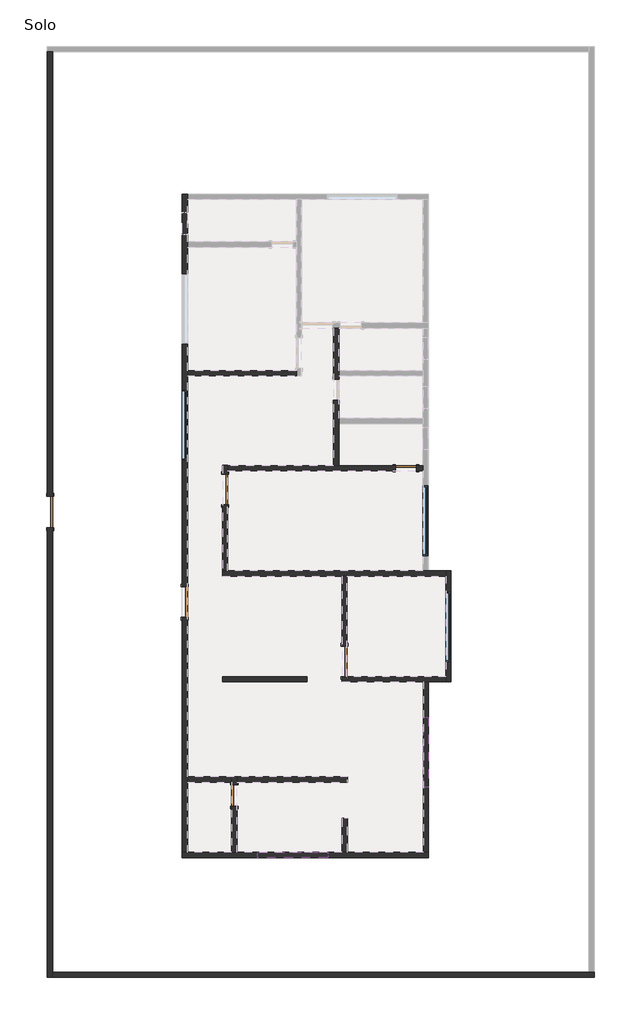
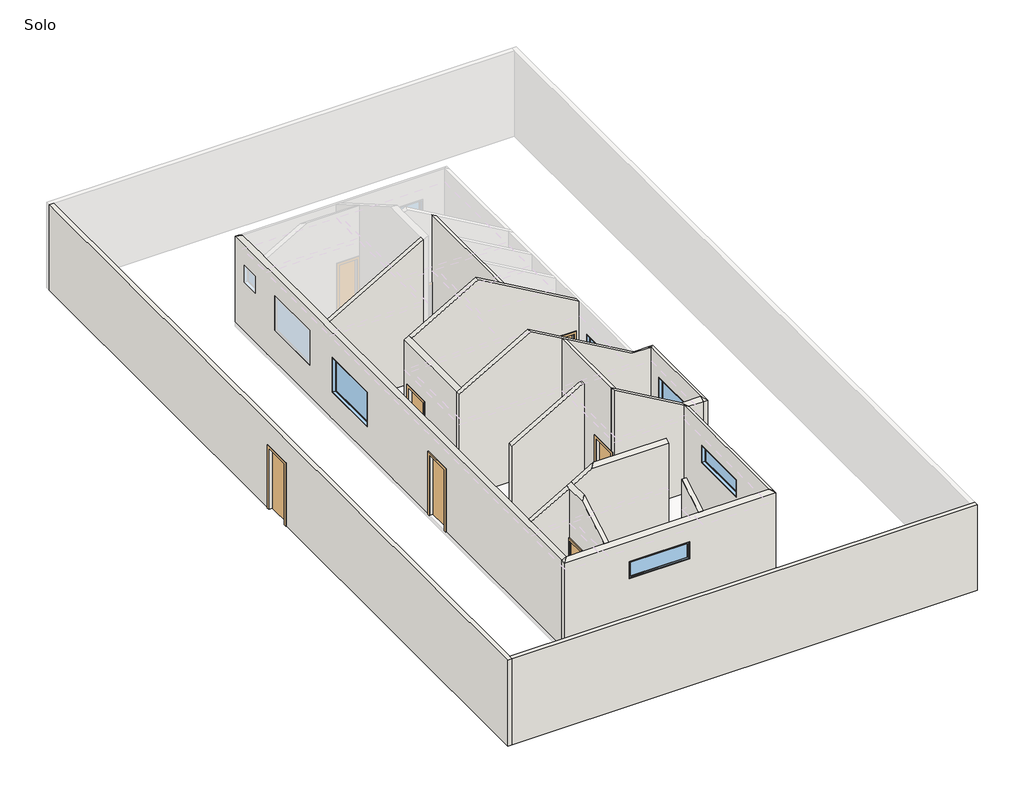
# One storey, part 1 of 2: 18 walls, 6 doors, 5 windows.
"""IFC4 building model written with IfcOpenShell, lengths in millimetres."""

import ifcopenshell
import ifcopenshell.guid

model = None  # the IFC model being written
_history = None  # IfcOwnerHistory: only IFC2X3 demands one
_inside = {}  # id of a spatial element -> (the spatial element, [elements in it])
_under = {}  # id of a project, library or spatial element -> (it, [spatial elements below it])
_declared = {}  # id of a project -> (the project, [libraries it declares])
_typed = {}  # id of a type object -> (the type object, [elements of that type])
_made_of = {}  # id of a material, layer set ... -> (it, [elements and type objects made of it])


def new_model(schema):
    """Start an empty IFC model of exactly this schema.

    Asked for "IFC4X3", IfcOpenShell would pick the latest addendum, in which some entities
    have other attributes; the version numbers below select the first issue.
    IFC2X3 requires an IfcOwnerHistory on every rooted entity: one is made here for all.
    """
    global model, _history
    if schema == "IFC4X3":
        model = ifcopenshell.file(schema_version=(4, 3, 0, 0))
    else:
        model = ifcopenshell.file(schema=schema)
    _inside.clear()
    _under.clear()
    _declared.clear()
    _typed.clear()
    _made_of.clear()
    _history = None
    if model.schema == "IFC2X3":
        org = make("IfcOrganization", Name="unknown")
        user = make(
            "IfcPersonAndOrganization",
            ThePerson=make("IfcPerson", FamilyName="unknown"),
            TheOrganization=org,
        )
        app = make(
            "IfcApplication",
            ApplicationDeveloper=org,
            Version="unknown",
            ApplicationFullName="unknown",
            ApplicationIdentifier="unknown",
        )
        _history = make(
            "IfcOwnerHistory",
            OwningUser=user,
            OwningApplication=app,
            ChangeAction="ADDED",
            CreationDate=0,
        )
    return model


def make(cls, **values):
    """One entity of the class cls with the attributes given. An attribute that is None is left unset."""
    return model.create_entity(
        cls, **{name: value for name, value in values.items() if value is not None}
    )


def rooted(cls, **values):
    """An entity with a GlobalId (a new one), such as an element, a storey or a relation."""
    return make(cls, GlobalId=ifcopenshell.guid.new(), OwnerHistory=_history, **values)


def si_unit(unit_type, name, prefix=None):
    """IfcSIUnit, for example si_unit("LENGTHUNIT", "METRE", prefix="MILLI")."""
    return make("IfcSIUnit", UnitType=unit_type, Prefix=prefix, Name=name)


def assignment(units):
    """IfcUnitAssignment: the units of a project."""
    return None if units is None else make("IfcUnitAssignment", Units=units)


def point(xyz):
    """IfcCartesianPoint."""
    return None if xyz is None else make("IfcCartesianPoint", Coordinates=xyz)


def direction(xyz):
    """IfcDirection."""
    return None if xyz is None else make("IfcDirection", DirectionRatios=xyz)


def frame(location, z_axis=None, x_axis=None):
    """IfcAxis2Placement3D, a coordinate frame: its origin and axes. An axis left out is left unset."""
    return make(
        "IfcAxis2Placement3D",
        Location=point(location),
        Axis=direction(z_axis),
        RefDirection=direction(x_axis),
    )


def origin():
    """The frame at (0, 0, 0) with its axes left unset."""
    return frame((0.0, 0.0, 0.0))


def origin_with_axes():
    """The frame at (0, 0, 0) with the z axis (0, 0, 1) and the x axis (1, 0, 0) written out."""
    return frame((0.0, 0.0, 0.0), z_axis=(0.0, 0.0, 1.0), x_axis=(1.0, 0.0, 0.0))


def place(relative_to, where):
    """IfcLocalPlacement: puts the frame where relative to a parent placement (None: the world)."""
    return make(
        "IfcLocalPlacement", PlacementRelTo=relative_to, RelativePlacement=where
    )


def context(
    kind, dimensions, precision=None, world=None, true_north=None, identifier=None
):
    """IfcGeometricRepresentationContext, for example the 3D "Model" context."""
    return make(
        "IfcGeometricRepresentationContext",
        ContextIdentifier=identifier,
        ContextType=kind,
        CoordinateSpaceDimension=dimensions,
        Precision=precision,
        WorldCoordinateSystem=world,
        TrueNorth=true_north,
    )


def project(units=None, contexts=None):
    """IfcProject with its units and contexts."""
    return rooted(
        "IfcProject",
        Name="project",
        RepresentationContexts=contexts,
        UnitsInContext=assignment(units),
    )


def spatial(cls, under=None, at=None, **own):
    """A site, building, storey or space (cls), placed at a placement, below another one or the project."""
    s = rooted(cls, ObjectPlacement=at, **own)
    if under is not None:
        _under.setdefault(under.id(), (under, []))[1].append(s)
    return s


def polyline(points):
    """IfcPolyline through the points."""
    return make("IfcPolyline", Points=[point(p) for p in points])


def outline(outer, holes=None, kind="AREA"):
    """IfcArbitraryClosedProfileDef: a profile drawn as a closed curve; with holes, ...WithVoids."""
    if holes is None:
        return make("IfcArbitraryClosedProfileDef", ProfileType=kind, OuterCurve=outer)
    return make(
        "IfcArbitraryProfileDefWithVoids",
        ProfileType=kind,
        OuterCurve=outer,
        InnerCurves=holes,
    )


def extrude(swept, where, along, depth):
    """IfcExtrudedAreaSolid: the profile swept, set in the frame where, extruded along a direction by depth."""
    return make(
        "IfcExtrudedAreaSolid",
        SweptArea=swept,
        Position=where,
        ExtrudedDirection=direction(along),
        Depth=depth,
    )


def faces_of(points, faces, orient=None, outer=None):
    """IfcFace entities. A face is a list of loops; a loop is a list of indices into points, from 0.

    orient and outer hold one flag for each loop. By default every Orientation is true, the
    first loop of a face is its IfcFaceOuterBound and the others are IfcFaceBound.
    """
    made = []
    for i, loops in enumerate(faces):
        bounds = []
        for j, loop in enumerate(loops):
            is_outer = j == 0 if outer is None else outer[i][j]
            bounds.append(
                make(
                    "IfcFaceOuterBound" if is_outer else "IfcFaceBound",
                    Bound=make("IfcPolyLoop", Polygon=[points[k] for k in loop]),
                    Orientation=True if orient is None else orient[i][j],
                )
            )
        made.append(make("IfcFace", Bounds=bounds))
    return made


def faceted_brep(points, faces, orient=None, outer=None, voids=None):
    """IfcFacetedBrep: a solid bounded by flat faces; with voids (closed shells), ...WithVoids."""
    shared = [point(p) for p in points]
    hull = make("IfcClosedShell", CfsFaces=faces_of(shared, faces, orient, outer))
    if voids is None:
        return make("IfcFacetedBrep", Outer=hull)
    return make(
        "IfcFacetedBrepWithVoids",
        Outer=hull,
        Voids=[
            make(cls, CfsFaces=faces_of(shared, fs, o, b)) for cls, fs, o, b in voids
        ],
    )


def shape(context_of_items, identifier, shape_type, items):
    """IfcShapeRepresentation: the items that make up one representation, for example the "Body"."""
    return make(
        "IfcShapeRepresentation",
        ContextOfItems=context_of_items,
        RepresentationIdentifier=identifier,
        RepresentationType=shape_type,
        Items=items,
    )


def source(mapping_origin, context_of_items, identifier, shape_type, items):
    """IfcRepresentationMap: a shape defined once, which mapped items show again and again."""
    return make(
        "IfcRepresentationMap",
        MappingOrigin=mapping_origin,
        MappedRepresentation=shape(context_of_items, identifier, shape_type, items),
    )


def transform(
    local_origin,
    x_axis=None,
    y_axis=None,
    z_axis=None,
    scale=None,
    scale2=None,
    scale3=None,
    uniform=True,
):
    """IfcCartesianTransformationOperator3D, or its non-uniform kind. x_axis, y_axis, z_axis: its Axis1, 2, 3."""
    if uniform:
        return make(
            "IfcCartesianTransformationOperator3D",
            Axis1=direction(x_axis),
            Axis2=direction(y_axis),
            LocalOrigin=point(local_origin),
            Scale=scale,
            Axis3=direction(z_axis),
        )
    return make(
        "IfcCartesianTransformationOperator3DnonUniform",
        Axis1=direction(x_axis),
        Axis2=direction(y_axis),
        LocalOrigin=point(local_origin),
        Scale=scale,
        Axis3=direction(z_axis),
        Scale2=scale2,
        Scale3=scale3,
    )


def mapped(mapping_source, mapping_target):
    """IfcMappedItem: shows the shape of a source again, moved by a transform."""
    return make(
        "IfcMappedItem", MappingSource=mapping_source, MappingTarget=mapping_target
    )


def made_of(thing, what):
    """Note that an element or type object is made of a material, layer set ...; save() writes the relation."""
    if what is not None:
        _made_of.setdefault(what.id(), (what, []))[1].append(thing)
    return thing


def element(
    cls,
    number,
    at=None,
    inside=None,
    cuts=None,
    type_object=None,
    material=None,
    context=None,
    identifier="Body",
    shape_type=None,
    held_by="IfcProductDefinitionShape",
    body=None,
    shapes=None,
    **own,
):
    """One element of the class cls, such as IfcWall. Its Tag is "e" and its number.

    at: its placement. inside: the storey or other place that contains it. cuts: it is an
    opening in that element (IfcRelVoidsElement). A single representation is given by context,
    identifier, shape_type and body (its items); several are given by shapes. held_by: the class
    of the entity that holds the representations. save() writes the other relations.
    """
    e = rooted(cls, Tag="e%d" % number, ObjectPlacement=at, **own)
    if body is not None:
        shapes = [shape(context, identifier, shape_type, body)]
    if shapes is not None:
        e.Representation = make(held_by, Representations=shapes)
    if inside is not None:
        _inside.setdefault(inside.id(), (inside, []))[1].append(e)
    if cuts is not None:
        rooted(
            "IfcRelVoidsElement", RelatingBuildingElement=cuts, RelatedOpeningElement=e
        )
    if type_object is not None:
        _typed.setdefault(type_object.id(), (type_object, []))[1].append(e)
    return made_of(e, material)


def aggregate(whole, parts):
    """IfcRelAggregates: a whole, such as a stair, and the parts it consists of."""
    return rooted("IfcRelAggregates", RelatingObject=whole, RelatedObjects=parts)


def save(model, path):
    """Write the relations noted so far, then the file.

    IfcRelAggregates (storeys below a building ...), IfcRelContainedInSpatialStructure (elements
    in a storey), IfcRelDefinesByType, IfcRelAssociatesMaterial and IfcRelDeclares: one each for
    every whole, place, type object, material and project.
    """
    for whole, parts in _under.values():
        aggregate(whole, parts)
    for where, things in _inside.values():
        rooted(
            "IfcRelContainedInSpatialStructure",
            RelatedElements=things,
            RelatingStructure=where,
        )
    for kind, things in _typed.values():
        rooted("IfcRelDefinesByType", RelatedObjects=things, RelatingType=kind)
    for what, things in _made_of.values():
        rooted("IfcRelAssociatesMaterial", RelatedObjects=things, RelatingMaterial=what)
    for by, libraries in _declared.values():
        rooted("IfcRelDeclares", RelatingContext=by, RelatedDefinitions=libraries)
    model.write(path)


def door_0762_x_2032mm_f712f77f(model_context):
    return source(origin(), model_context, "Body", "SweptSolid", [
        extrude(outline(polyline([(2108.0, -376.0), (0.0, -376.0), (0.0, -300.0), (2032.0, -300.0), (2032.0, 300.0), (0.0, 300.0), (0.0, 376.0), (2108.0, 376.0), (2108.0, -376.0)])), frame((0.0, 75.0, 0.0), z_axis=(0.0, 1.0, 0.0), x_axis=(0.0, 0.0, 1.0)), (0.0, 0.0, 1.0), 25.0),
        extrude(outline(polyline([(2108.0, 376.0), (2108.0, -376.0), (0.0, -376.0), (0.0, -300.0), (2032.0, -300.0), (2032.0, 300.0), (0.0, 300.0), (0.0, 376.0), (2108.0, 376.0)])), frame((0.0, -100.0, 0.0), z_axis=(0.0, 1.0, 0.0), x_axis=(0.0, 0.0, 1.0)), (0.0, 0.0, 1.0), 25.0),
        extrude(outline(polyline([(300.0, 24.0), (-300.0, 24.0), (-300.0, 75.0), (300.0, 75.0), (300.0, 24.0)])), origin_with_axes(), (0.0, 0.0, 1.0), 2032.0),
    ])


def door_0864_x_2134mm_0748c0c9(model_context):
    return source(origin(), model_context, "Body", "SweptSolid", [
        extrude(outline(polyline([(2210.0, -508.0), (0.0, -508.0), (0.0, -432.0), (2134.0, -432.0), (2134.0, 432.0), (0.0, 432.0), (0.0, 508.0), (2210.0, 508.0), (2210.0, -508.0)])), frame((0.0, -100.0, 0.0), z_axis=(0.0, 1.0, 0.0), x_axis=(0.0, 0.0, 1.0)), (0.0, 0.0, 1.0), 25.0),
        extrude(outline(polyline([(2210.0, 508.0), (2210.0, -508.0), (0.0, -508.0), (0.0, -432.0), (2134.0, -432.0), (2134.0, 432.0), (0.0, 432.0), (0.0, 508.0), (2210.0, 508.0)])), frame((0.0, 75.0, 0.0), z_axis=(0.0, 1.0, 0.0), x_axis=(0.0, 0.0, 1.0)), (0.0, 0.0, 1.0), 25.0),
        extrude(outline(polyline([(432.0, -24.0), (432.0, -75.0), (-432.0, -75.0), (-432.0, -24.0), (432.0, -24.0)])), origin_with_axes(), (0.0, 0.0, 1.0), 2134.0),
    ])


def door_0864_x_2134mm_191ab4f9(model_context):
    return source(origin(), model_context, "Body", "SweptSolid", [
        extrude(outline(polyline([(2210.0, -508.0), (0.0, -508.0), (0.0, -432.0), (2134.0, -432.0), (2134.0, 432.0), (0.0, 432.0), (0.0, 508.0), (2210.0, 508.0), (2210.0, -508.0)])), frame((0.0, 75.0, 0.0), z_axis=(0.0, 1.0, 0.0), x_axis=(0.0, 0.0, 1.0)), (0.0, 0.0, 1.0), 25.0),
        extrude(outline(polyline([(2210.0, 508.0), (2210.0, -508.0), (0.0, -508.0), (0.0, -432.0), (2134.0, -432.0), (2134.0, 432.0), (0.0, 432.0), (0.0, 508.0), (2210.0, 508.0)])), frame((0.0, -100.0, 0.0), z_axis=(0.0, 1.0, 0.0), x_axis=(0.0, 0.0, 1.0)), (0.0, 0.0, 1.0), 25.0),
        extrude(outline(polyline([(432.0, 24.0), (-432.0, 24.0), (-432.0, 75.0), (432.0, 75.0), (432.0, 24.0)])), origin_with_axes(), (0.0, 0.0, 1.0), 2134.0),
    ])


def door_0915_x_2134mm_ecbf01f7(model_context):
    return source(origin(), model_context, "Body", "SweptSolid", [
        extrude(outline(polyline([(2210.0, -526.0), (0.0, -526.0), (0.0, -450.0), (2134.0, -450.0), (2134.0, 450.0), (0.0, 450.0), (0.0, 526.0), (2210.0, 526.0), (2210.0, -526.0)])), frame((0.0, 75.0, 0.0), z_axis=(0.0, 1.0, 0.0), x_axis=(0.0, 0.0, 1.0)), (0.0, 0.0, 1.0), 25.0),
        extrude(outline(polyline([(2210.0, 526.0), (2210.0, -526.0), (0.0, -526.0), (0.0, -450.0), (2134.0, -450.0), (2134.0, 450.0), (0.0, 450.0), (0.0, 526.0), (2210.0, 526.0)])), frame((0.0, -100.0, 0.0), z_axis=(0.0, 1.0, 0.0), x_axis=(0.0, 0.0, 1.0)), (0.0, 0.0, 1.0), 25.0),
        extrude(outline(polyline([(450.0, 24.0), (-450.0, 24.0), (-450.0, 75.0), (450.0, 75.0), (450.0, 24.0)])), origin_with_axes(), (0.0, 0.0, 1.0), 2134.0),
    ])


def m_fixo_0915_x_0610mm_568dc35f(model_context):
    return source(origin(), model_context, "Body", "SweptSolid", [
        extrude(outline(polyline([(-937.0, 53.0), (937.0, 53.0), (937.0, 41.0), (-937.0, 41.0), (-937.0, 53.0)])), frame((0.0, 0.0, 2063.0), z_axis=(0.0, 0.0, 1.0), x_axis=(1.0, 0.0, 0.0)), (0.0, 0.0, 1.0), 484.0),
        extrude(outline(polyline([(2591.0, -981.0), (2019.0, -981.0), (2019.0, 981.0), (2591.0, 981.0), (2591.0, -981.0)]), holes=[polyline([(2547.0, -937.0), (2547.0, 937.0), (2063.0, 937.0), (2063.0, -937.0), (2547.0, -937.0)])]), frame((0.0, 25.0, 0.0), z_axis=(0.0, 1.0, 0.0), x_axis=(0.0, 0.0, 1.0)), (0.0, 0.0, 1.0), 44.0),
        extrude(outline(polyline([(2610.0, -1000.0), (2000.0, -1000.0), (2000.0, 1000.0), (2610.0, 1000.0), (2610.0, -1000.0)]), holes=[polyline([(2591.0, -981.0), (2591.0, 981.0), (2019.0, 981.0), (2019.0, -981.0), (2591.0, -981.0)])]), frame((0.0, 25.0, 0.0), z_axis=(0.0, 1.0, 0.0), x_axis=(0.0, 0.0, 1.0)), (0.0, 0.0, 1.0), 63.0),
        extrude(outline(polyline([(2610.0, -1000.0), (2000.0, -1000.0), (2000.0, 1000.0), (2610.0, 1000.0), (2610.0, -1000.0)]), holes=[polyline([(2578.0, -968.0), (2578.0, 968.0), (2032.0, 968.0), (2032.0, -968.0), (2578.0, -968.0)])]), frame((0.0, -62.0, 0.0), z_axis=(0.0, 1.0, 0.0), x_axis=(0.0, 0.0, 1.0)), (0.0, 0.0, 1.0), 87.0),
    ])


def m_fixo_0915_x_1220mm_8e554ddc(model_context):
    return source(origin(), model_context, "Body", "SweptSolid", [
        extrude(outline(polyline([(-937.0, 53.0), (937.0, 53.0), (937.0, 41.0), (-937.0, 41.0), (-937.0, 53.0)])), frame((0.0, 0.0, 978.0), z_axis=(0.0, 0.0, 1.0), x_axis=(1.0, 0.0, 0.0)), (0.0, 0.0, 1.0), 1094.0),
        extrude(outline(polyline([(2116.0, -981.0), (934.0, -981.0), (934.0, 981.0), (2116.0, 981.0), (2116.0, -981.0)]), holes=[polyline([(2072.0, -937.0), (2072.0, 937.0), (978.0, 937.0), (978.0, -937.0), (2072.0, -937.0)])]), frame((0.0, 25.0, 0.0), z_axis=(0.0, 1.0, 0.0), x_axis=(0.0, 0.0, 1.0)), (0.0, 0.0, 1.0), 44.0),
        extrude(outline(polyline([(2135.0, -1000.0), (915.0, -1000.0), (915.0, 1000.0), (2135.0, 1000.0), (2135.0, -1000.0)]), holes=[polyline([(2116.0, -981.0), (2116.0, 981.0), (934.0, 981.0), (934.0, -981.0), (2116.0, -981.0)])]), frame((0.0, 25.0, 0.0), z_axis=(0.0, 1.0, 0.0), x_axis=(0.0, 0.0, 1.0)), (0.0, 0.0, 1.0), 63.0),
        extrude(outline(polyline([(2135.0, -1000.0), (915.0, -1000.0), (915.0, 1000.0), (2135.0, 1000.0), (2135.0, -1000.0)]), holes=[polyline([(2103.0, -968.0), (2103.0, 968.0), (947.0, 968.0), (947.0, -968.0), (2103.0, -968.0)])]), frame((0.0, -62.0, 0.0), z_axis=(0.0, 1.0, 0.0), x_axis=(0.0, 0.0, 1.0)), (0.0, 0.0, 1.0), 87.0),
    ])


model = new_model("IFC4")

# Units and contexts
model_context = context("Model", 3, world=origin())
ifc_project = project(units=[si_unit("LENGTHUNIT", "METRE", prefix="MILLI")], contexts=[model_context])

# Site, building, storey
site = spatial("IfcSite", under=ifc_project)
building = spatial("IfcBuilding", under=site)
storey = spatial("IfcBuildingStorey", under=building, Name="Solo", Elevation=0.0)

# Doors
placement = place(None, origin())
door_0762_x_2032mm_shape = door_0762_x_2032mm_f712f77f(model_context)
element("IfcDoor", 1, ObjectType="M_Folha única : 0762 x 2032mm", at=placement, inside=storey, context=model_context, shape_type="MappedRepresentation", body=[
    mapped(door_0762_x_2032mm_shape, transform((-4950.9149651, -8006.6262329, 0.0), x_axis=(0.0, 1.0, 0.0), y_axis=(-1.0, 0.0, 0.0), z_axis=(0.0, 0.0, 1.0))),
])
element("IfcDoor", 2, ObjectType="M_Folha única : 0762 x 2032mm", at=placement, inside=storey, context=model_context, shape_type="MappedRepresentation", body=[
    mapped(door_0762_x_2032mm_shape, transform((-70.8698769, 1295.0972582, 0.0), x_axis=(1.0, 0.0, 0.0), y_axis=(0.0, 1.0, 0.0), z_axis=(0.0, 0.0, 1.0))),
])
door_0864_x_2134mm_shape = door_0864_x_2134mm_0748c0c9(model_context)
element("IfcDoor", 3, ObjectType="M_Folha única : 0864 x 2134mm", at=placement, inside=storey, context=model_context, shape_type="MappedRepresentation", body=[
    mapped(door_0864_x_2134mm_shape, transform((-5214.335632, 688.0972582, 0.0), x_axis=(0.0, 1.0, 0.0), y_axis=(-1.0, 0.0, 0.0), z_axis=(0.0, 0.0, 1.0))),
])
element("IfcDoor", 4, ObjectType="M_Folha única : 0864 x 2134mm", at=placement, inside=storey, context=model_context, shape_type="MappedRepresentation", body=[
    mapped(door_0864_x_2134mm_shape, transform((-6360.8698767, -2511.9027414, 0.0), x_axis=(0.0, 1.0, 0.0), y_axis=(-1.0, 0.0, 0.0), z_axis=(0.0, 0.0, 1.0))),
])
door_0864_x_2134mm_2_shape = door_0864_x_2134mm_191ab4f9(model_context)
element("IfcDoor", 5, ObjectType="M_Folha única : 0864 x 2134mm", at=placement, inside=storey, context=model_context, shape_type="MappedRepresentation", body=[
    mapped(door_0864_x_2134mm_2_shape, transform((-1820.8247891, -4192.9027402, 0.0), x_axis=(0.0, -1.0, 0.0), y_axis=(1.0, 0.0, 0.0), z_axis=(0.0, 0.0, 1.0))),
])
door_0915_x_2134mm_shape = door_0915_x_2134mm_ecbf01f7(model_context)
element("IfcDoor", 6, ObjectType="M_Folha única : 0915 x 2134mm", at=placement, inside=storey, context=model_context, shape_type="MappedRepresentation", body=[
    mapped(door_0915_x_2134mm_shape, transform((-10190.8698769, 50.0972598, 0.0), x_axis=(0.0, -1.0, 0.0), y_axis=(1.0, 0.0, 0.0), z_axis=(0.0, 0.0, 1.0))),
])

# Walls
element("IfcWall", 7, ObjectType="Genérico - 140 mm Alvenaria", at=placement, inside=storey, context=model_context, shape_type="Brep", body=[
    faceted_brep([(574.1301232, -9623.7945276, 0.0), (424.1301232, -9623.7945276, 0.0), (-1735.8698771, -9623.7945276, 0.0), (-1885.8698771, -9623.7945276, 0.0), (-4875.9149651, -9623.7945276, 0.0), (-5025.9149651, -9623.7945276, 0.0), (-6285.8698767, -9623.7945276, 0.0), (-6435.8698767, -9623.7945276, 0.0), (-6435.8698767, -9623.7945276, 3000.0), (-6285.8698767, -9623.7945276, 3086.6025404), (-5025.9149651, -9623.7945276, 3086.6025404), (-4875.9149651, -9623.7945276, 3086.6025404), (-1885.8698771, -9623.7945276, 3086.6025404), (-1735.8698771, -9623.7945276, 3086.6025404), (424.1301232, -9623.7945276, 3086.6025404), (574.1301232, -9623.7945276, 3000.0), (-2285.8698771, -9623.7945276, 1690.0), (-2285.8698771, -9623.7945276, 2300.0), (-4285.8698771, -9623.7945276, 2300.0), (-4285.8698771, -9623.7945276, 1690.0), (574.1301232, -9773.7945276, 0.0), (574.1301232, -9773.7945276, 3000.0), (-6435.8698767, -9773.7945276, 3000.0), (-6435.8698767, -9773.7945276, 0.0), (-2285.8698771, -9773.7945276, 1690.0), (-4285.8698771, -9773.7945276, 1690.0), (-4285.8698771, -9773.7945276, 2300.0), (-2285.8698771, -9773.7945276, 2300.0)], [[[0, 1, 2, 3, 4, 5, 6, 7, 8, 9, 10, 11, 12, 13, 14, 15], [16, 17, 18, 19]], [[20, 21, 22, 23], [24, 25, 26, 27]], [[7, 6, 5, 4, 3, 2, 1, 0, 20, 23]], [[8, 7, 23, 22]], [[0, 15, 21, 20]], [[17, 16, 24, 27]], [[18, 17, 27, 26]], [[19, 18, 26, 25]], [[16, 19, 25, 24]], [[15, 14, 21]], [[14, 13, 12, 11, 10, 9, 22, 21]], [[9, 8, 22]]]),
])
element("IfcWall", 8, ObjectType="Genérico - 140 mm Alvenaria", at=placement, inside=storey, context=model_context, shape_type="Brep", body=[
    faceted_brep([(-5025.9149651, -7474.9027402, 0.0), (-5025.9149651, -7476.6262329, 0.0), (-5025.9149651, -7626.6262329, 0.0), (-5025.9149651, -7706.6262329, 0.0), (-5025.9149651, -7706.6262329, 2032.0), (-5025.9149651, -8306.6262329, 2032.0), (-5025.9149651, -8306.6262329, 0.0), (-5025.9149651, -9623.7945276, 0.0), (-5025.9149651, -9623.7945276, 3086.6025404), (-5025.9149651, -8363.839616, 3814.0378477), (-5025.9149651, -7626.6262329, 3814.0378477), (-5025.9149651, -7476.6262329, 3814.0378477), (-5025.9149651, -7474.9027402, 3814.0378477), (-4875.9149651, -7706.6262329, 2032.0), (-4875.9149651, -7706.6262329, 0.0), (-4875.9149651, -7626.6262329, 0.0), (-4875.9149651, -7476.6262329, 0.0), (-4875.9149651, -7474.9027402, 0.0), (-4875.9149651, -7474.9027402, 3900.6403881), (-4875.9149651, -7476.6262329, 3900.6403881), (-4875.9149651, -7626.6262329, 3900.6403881), (-4875.9149651, -8213.839616, 3900.6403881), (-4875.9149651, -9623.7945276, 3086.6025404), (-4875.9149651, -9623.7945276, 0.0), (-4875.9149651, -8306.6262329, 0.0), (-4875.9149651, -8306.6262329, 2032.0)], [[[0, 1, 2, 3, 4, 5, 6, 7, 8, 9, 10, 11, 12]], [[13, 14, 15, 16, 17, 18, 19, 20, 21, 22, 23, 24, 25]], [[24, 23, 7, 6]], [[17, 16, 15, 14, 3, 2, 1, 0]], [[0, 12, 18, 17]], [[8, 7, 23, 22]], [[4, 3, 14, 13]], [[5, 4, 13, 25]], [[6, 5, 25, 24]], [[12, 11, 10, 9, 21, 20, 19, 18]], [[9, 8, 22, 21]]]),
])
element("IfcWall", 9, ObjectType="Genérico - 140 mm Alvenaria", at=placement, inside=storey, context=model_context, shape_type="Brep", body=[
    faceted_brep([(-4875.9149651, -7626.6262329, 0.0), (-1735.8698771, -7626.6262329, 0.0), (-1735.8698771, -7626.6262329, 4239.6681929), (-4288.7015821, -7626.6262329, 4239.6681929), (-4875.9149651, -7626.6262329, 3900.6403881), (-4875.9149651, -7476.6262329, 0.0), (-4875.9149651, -7476.6262329, 3900.6403881), (-4138.7015821, -7476.6262329, 4326.2707333), (-1735.8698771, -7476.6262329, 4326.2707333), (-1735.8698771, -7476.6262329, 0.0)], [[[0, 1, 2, 3, 4]], [[5, 6, 7, 8, 9]], [[1, 0, 5, 9]], [[2, 1, 9, 8]], [[0, 4, 6, 5]], [[4, 3, 7, 6]], [[3, 2, 8, 7]]]),
])
element("IfcWall", 10, ObjectType="Genérico - 140 mm Alvenaria", at=placement, inside=storey, context=model_context, shape_type="SweptSolid", body=[
    extrude(outline(polyline([(-8644.9027402, 0.0), (-9623.7945276, 0.0), (-9623.7945276, 3086.6025404), (-8644.9027402, 3651.7659773), (-8644.9027402, 0.0)])), frame((-1885.8698771, 0.0, 0.0), z_axis=(1.0, 0.0, 0.0), x_axis=(0.0, 1.0, 0.0)), (0.0, 0.0, 1.0), 150.0),
])
element("IfcWall", 11, ObjectType="Genérico - 140 mm Alvenaria", at=placement, inside=storey, context=model_context, shape_type="SweptSolid", body=[
    extrude(outline(polyline([(0.0, -6285.8698767), (0.0, -5025.9149651), (3814.0378477, -5025.9149651), (3086.6025404, -6285.8698767), (0.0, -6285.8698767)])), frame((0.0, -7626.6262329, 0.0), z_axis=(0.0, 1.0, 0.0), x_axis=(0.0, 0.0, 1.0)), (0.0, 0.0, 1.0), 150.0),
])
element("IfcWall", 12, ObjectType="Genérico - 140 mm Alvenaria", at=placement, inside=storey, context=model_context, shape_type="Brep", body=[
    faceted_brep([(-6285.8698767, -2079.9027414, 2134.0), (-6285.8698767, -2079.9027414, 0.0), (-6285.8698767, 3920.0972586, 0.0), (-6285.8698767, 4070.0972586, 0.0), (-6285.8698767, 7575.0972586, 0.0), (-6285.8698767, 7725.0972586, 0.0), (-6285.8698767, 8932.5972586, 0.0), (-6285.8698767, 9082.5972586, 0.0), (-6285.8698767, 9082.5972586, 3000.0), (-6285.8698767, 8932.5972586, 3086.6025404), (-6285.8698767, 7725.0972586, 3086.6025404), (-6285.8698767, 7575.0972586, 3086.6025404), (-6285.8698767, 4070.0972586, 3086.6025404), (-6285.8698767, 3920.0972586, 3086.6025404), (-6285.8698767, -7476.6262329, 3086.6025404), (-6285.8698767, -7626.6262329, 3086.6025404), (-6285.8698767, -9623.7945276, 3086.6025404), (-6285.8698767, -9623.7945276, 0.0), (-6285.8698767, -7626.6262329, 0.0), (-6285.8698767, -7476.6262329, 0.0), (-6285.8698767, -2943.9027414, 0.0), (-6285.8698767, -2943.9027414, 2134.0), (-6285.8698767, 8572.5972586, 1700.0), (-6285.8698767, 7932.5972586, 1700.0), (-6285.8698767, 7932.5972586, 2300.0), (-6285.8698767, 8572.5972586, 2300.0), (-6285.8698767, 4822.5972586, 1080.5823766), (-6285.8698767, 4822.5972586, 2300.5823766), (-6285.8698767, 6822.5972586, 2300.5823766), (-6285.8698767, 6822.5972586, 1080.5823766), (-6285.8698767, 3520.0972586, 915.0), (-6285.8698767, 1520.0972586, 915.0), (-6285.8698767, 1520.0972586, 2135.0), (-6285.8698767, 3520.0972586, 2135.0), (-6435.8698767, 9082.5972586, 0.0), (-6435.8698767, -2079.9027414, 0.0), (-6435.8698767, -2079.9027414, 2134.0), (-6435.8698767, -2943.9027414, 2134.0), (-6435.8698767, -2943.9027414, 0.0), (-6435.8698767, -9623.7945276, 0.0), (-6435.8698767, -9623.7945276, 3000.0), (-6435.8698767, 9082.5972586, 3000.0), (-6435.8698767, 8572.5972586, 1700.0), (-6435.8698767, 8572.5972586, 2300.0), (-6435.8698767, 7932.5972586, 2300.0), (-6435.8698767, 7932.5972586, 1700.0), (-6435.8698767, 4822.5972586, 1080.5823766), (-6435.8698767, 6822.5972586, 1080.5823766), (-6435.8698767, 6822.5972586, 2300.5823766), (-6435.8698767, 4822.5972586, 2300.5823766), (-6435.8698767, 3520.0972586, 915.0), (-6435.8698767, 3520.0972586, 2135.0), (-6435.8698767, 1520.0972586, 2135.0), (-6435.8698767, 1520.0972586, 915.0)], [[[0, 1, 2, 3, 4, 5, 6, 7, 8, 9, 10, 11, 12, 13, 14, 15, 16, 17, 18, 19, 20, 21], [22, 23, 24, 25], [26, 27, 28, 29], [30, 31, 32, 33]], [[34, 35, 36, 37, 38, 39, 40, 41], [42, 43, 44, 45], [46, 47, 48, 49], [50, 51, 52, 53]], [[7, 6, 5, 4, 3, 2, 1, 35, 34]], [[20, 19, 18, 17, 39, 38]], [[17, 16, 40, 39]], [[8, 7, 34, 41]], [[43, 42, 22, 25]], [[44, 43, 25, 24]], [[45, 44, 24, 23]], [[42, 45, 23, 22]], [[27, 26, 46, 49]], [[28, 27, 49, 48]], [[29, 28, 48, 47]], [[26, 29, 47, 46]], [[51, 50, 30, 33]], [[52, 51, 33, 32]], [[53, 52, 32, 31]], [[50, 53, 31, 30]], [[36, 35, 1, 0]], [[37, 36, 0, 21]], [[38, 37, 21, 20]], [[16, 15, 14, 13, 12, 11, 10, 9, 41, 40]], [[9, 8, 41]]]),
])
element("IfcWall", 13, ObjectType="Genérico - 140 mm Alvenaria", at=placement, inside=storey, context=model_context, shape_type="SweptSolid", body=[
    extrude(outline(polyline([(0.0, -3187.4041224), (4875.5025777, -3187.4041224), (3086.6025404, -6285.8698767), (0.0, -6285.8698767), (0.0, -3187.4041224)])), frame((0.0, 3920.0972586, 0.0), z_axis=(0.0, 1.0, 0.0), x_axis=(0.0, 0.0, 1.0)), (0.0, 0.0, 1.0), 150.0),
])
element("IfcWall", 14, ObjectType="Genérico - 140 mm Alvenaria", at=placement, inside=storey, context=model_context, shape_type="Brep", body=[
    faceted_brep([(1059.1301231, -1624.902741, 0.0), (1059.1301231, -1774.902741, 0.0), (1059.1301231, -4624.9027402, 0.0), (1059.1301231, -4774.9027402, 0.0), (1059.1301231, -4774.9027402, 3000.0), (1059.1301231, -4624.9027402, 3086.6025404), (1059.1301231, -1774.902741, 3086.6025404), (1059.1301231, -1624.902741, 3000.0), (1059.1301231, -2214.902741, 1080.0), (1059.1301231, -2214.902741, 2300.0), (1059.1301231, -4214.902741, 2300.0), (1059.1301231, -4214.902741, 1080.0), (1209.1301231, -1624.902741, 0.0), (1209.1301231, -1624.902741, 3000.0), (1209.1301231, -4774.9027402, 3000.0), (1209.1301231, -4774.9027402, 0.0), (1209.1301231, -2214.902741, 1080.0), (1209.1301231, -4214.902741, 1080.0), (1209.1301231, -4214.902741, 2300.0), (1209.1301231, -2214.902741, 2300.0)], [[[0, 1, 2, 3, 4, 5, 6, 7], [8, 9, 10, 11]], [[12, 13, 14, 15], [16, 17, 18, 19]], [[3, 2, 1, 0, 12, 15]], [[4, 3, 15, 14]], [[0, 7, 13, 12]], [[9, 8, 16, 19]], [[10, 9, 19, 18]], [[11, 10, 18, 17]], [[8, 11, 17, 16]], [[7, 6, 13]], [[6, 5, 14, 13]], [[5, 4, 14]]]),
])
element("IfcWall", 15, ObjectType="Genérico - 140 mm Alvenaria", at=placement, inside=storey, context=model_context, shape_type="Brep", body=[
    faceted_brep([(-1895.8247891, -4774.9027402, 0.0), (424.1301232, -4774.9027402, 0.0), (574.1301232, -4774.9027402, 0.0), (1059.1301231, -4774.9027402, 0.0), (1059.1301231, -4774.9027402, 3000.0), (574.1301232, -4774.9027402, 3000.0), (424.1301232, -4774.9027402, 3086.6025404), (-1895.8247891, -4774.9027402, 4426.0291335), (-1895.8247891, -4624.9027402, 0.0), (-1895.8247891, -4624.9027402, 2134.0), (-1895.8247891, -4624.9027402, 4426.0291335), (-1745.8247891, -4624.9027402, 4339.4265931), (424.1301232, -4624.9027402, 3086.6025404), (1059.1301231, -4624.9027402, 3086.6025404), (1059.1301231, -4624.9027402, 0.0)], [[[0, 1, 2, 3, 4, 5, 6, 7]], [[8, 9, 10, 11, 12, 13, 14]], [[3, 2, 1, 0, 8, 14]], [[4, 3, 14, 13]], [[0, 7, 10, 9, 8]], [[7, 6, 5, 12, 11, 10]], [[5, 4, 13, 12]]]),
])
element("IfcWall", 16, ObjectType="Genérico - 140 mm Alvenaria", at=placement, inside=storey, context=model_context, shape_type="Brep", body=[
    faceted_brep([(-1895.8247891, -1774.902741, 4426.0291335), (-1895.8247891, -1774.902741, 0.0), (-1895.8247891, -3760.9027402, 0.0), (-1895.8247891, -3760.9027402, 2134.0), (-1895.8247891, -4624.9027402, 2134.0), (-1895.8247891, -4624.9027402, 4426.0291335), (-1745.8247891, -1774.902741, 0.0), (-1745.8247891, -1774.902741, 4339.4265931), (-1745.8247891, -4624.9027402, 4339.4265931), (-1745.8247891, -4624.9027402, 2134.0), (-1745.8247891, -3760.9027402, 2134.0), (-1745.8247891, -3760.9027402, 0.0)], [[[0, 1, 2, 3, 4, 5]], [[6, 7, 8, 9, 10, 11]], [[1, 6, 11, 2]], [[8, 5, 4, 9]], [[1, 0, 7, 6]], [[3, 10, 9, 4]], [[10, 3, 2, 11]], [[0, 5, 8, 7]]]),
])
element("IfcWall", 17, ObjectType="Genérico - 140 mm Alvenaria", at=placement, inside=storey, context=model_context, shape_type="Brep", body=[
    faceted_brep([(1059.1301231, -1624.902741, 0.0), (559.1301231, -1624.902741, 0.0), (409.1301231, -1624.902741, 0.0), (-5139.335632, -1624.902741, 0.0), (-5289.335632, -1624.902741, 0.0), (-5290.8698769, -1624.902741, 0.0), (-5290.8698769, -1624.902741, 3661.0660581), (-5289.335632, -1624.902741, 3661.9518548), (-5139.335632, -1624.902741, 3748.5543952), (-2930.8698768, -1624.902741, 5023.6126935), (409.1301231, -1624.902741, 3095.2627944), (559.1301231, -1624.902741, 3008.6602541), (574.1301232, -1624.902741, 3000.0), (1059.1301231, -1624.902741, 3000.0), (1059.1301231, -1774.902741, 0.0), (1059.1301231, -1774.902741, 3086.6025404), (424.1301232, -1774.902741, 3086.6025404), (-1745.8247891, -1774.902741, 4339.4265931), (-1895.8247891, -1774.902741, 4426.0291335), (-2930.8698768, -1774.902741, 5023.6126935), (-5290.8698769, -1774.902741, 3661.0660581), (-5290.8698769, -1774.902741, 0.0), (-1895.8247891, -1774.902741, 0.0), (-1745.8247891, -1774.902741, 0.0)], [[[0, 1, 2, 3, 4, 5, 6, 7, 8, 9, 10, 11, 12, 13]], [[14, 15, 16, 17, 18, 19, 20, 21, 22, 23]], [[5, 4, 3, 2, 1, 0, 14, 23, 22, 21]], [[6, 5, 21, 20]], [[0, 13, 15, 14]], [[13, 12, 16, 15]], [[12, 11, 10, 9, 19, 18, 17, 16]], [[9, 8, 7, 6, 20, 19]]]),
])
element("IfcWall", 18, ObjectType="Genérico - 140 mm Alvenaria", at=placement, inside=storey, context=model_context, shape_type="Brep", body=[
    faceted_brep([(-5139.335632, 1120.0972582, 2134.0), (-5139.335632, 1120.0972582, 0.0), (-5139.335632, 1220.0972582, 0.0), (-5139.335632, 1370.0972582, 0.0), (-5139.335632, 1375.097259, 0.0), (-5139.335632, 1375.097259, 3748.5543952), (-5139.335632, 1370.0972582, 3748.5543952), (-5139.335632, 1220.0972582, 3748.5543952), (-5139.335632, -1624.902741, 3748.5543952), (-5139.335632, -1624.902741, 0.0), (-5139.335632, 256.0972582, 0.0), (-5139.335632, 256.0972582, 2134.0), (-5289.335632, 1375.097259, 0.0), (-5289.335632, 1120.0972582, 0.0), (-5289.335632, 1120.0972582, 2134.0), (-5289.335632, 256.0972582, 2134.0), (-5289.335632, 256.0972582, 0.0), (-5289.335632, -1624.902741, 0.0), (-5289.335632, -1624.902741, 3661.9518548), (-5289.335632, 1375.097259, 3661.9518548)], [[[0, 1, 2, 3, 4, 5, 6, 7, 8, 9, 10, 11]], [[12, 13, 14, 15, 16, 17, 18, 19]], [[10, 9, 17, 16]], [[4, 3, 2, 1, 13, 12]], [[5, 4, 12, 19]], [[9, 8, 18, 17]], [[14, 13, 1, 0]], [[15, 14, 0, 11]], [[16, 15, 11, 10]], [[8, 7, 6, 5, 19, 18]]]),
])
element("IfcWall", 19, ObjectType="Genérico - 140 mm Alvenaria", at=placement, inside=storey, context=model_context, shape_type="Brep", body=[
    faceted_brep([(229.1301231, 1220.0972582, 2032.0), (229.1301231, 1220.0972582, 0.0), (409.1301231, 1220.0972582, 0.0), (409.1301231, 1220.0972582, 3095.2627944), (-2930.8698768, 1220.0972582, 5023.6126935), (-5139.335632, 1220.0972582, 3748.5543952), (-5139.335632, 1220.0972582, 0.0), (-370.8698769, 1220.0972582, 0.0), (-370.8698769, 1220.0972582, 2032.0), (409.1301231, 1370.0972582, 0.0), (229.1301231, 1370.0972582, 0.0), (229.1301231, 1370.0972582, 2032.0), (-370.8698769, 1370.0972582, 2032.0), (-370.8698769, 1370.0972582, 0.0), (-1979.4742231, 1370.0972582, 0.0), (-2129.4742231, 1370.0972582, 0.0), (-5139.335632, 1370.0972582, 0.0), (-5139.335632, 1370.0972582, 3748.5543952), (-2930.8698768, 1370.0972582, 5023.6126935), (-2129.4742231, 1370.0972582, 4560.9266971), (-1979.4742231, 1370.0972582, 4474.3241567), (409.1301231, 1370.0972582, 3095.2627944)], [[[0, 1, 2, 3, 4, 5, 6, 7, 8]], [[9, 10, 11, 12, 13, 14, 15, 16, 17, 18, 19, 20, 21]], [[7, 6, 16, 15, 14, 13]], [[2, 1, 10, 9]], [[3, 2, 9, 21]], [[6, 5, 17, 16]], [[11, 10, 1, 0]], [[12, 11, 0, 8]], [[13, 12, 8, 7]], [[5, 4, 18, 17]], [[4, 3, 21, 20, 19, 18]]]),
])
element("IfcWall", 20, ObjectType="Genérico - 140 mm Alvenaria", at=placement, inside=storey, context=model_context, shape_type="Brep", body=[
    faceted_brep([(-1979.4742231, 3820.0972586, 2032.0), (-1979.4742231, 3820.0972586, 0.0), (-1979.4742231, 3920.0972586, 0.0), (-1979.4742231, 4070.0972586, 0.0), (-1979.4742231, 5273.5630139, 0.0), (-1979.4742231, 5273.5630139, 4474.3241567), (-1979.4742231, 4070.0972586, 4474.3241567), (-1979.4742231, 3920.0972586, 4474.3241567), (-1979.4742231, 2713.9475745, 4474.3241567), (-1979.4742231, 2563.9475745, 4474.3241567), (-1979.4742231, 1370.0972582, 4474.3241567), (-1979.4742231, 1370.0972582, 0.0), (-1979.4742231, 2563.9475745, 0.0), (-1979.4742231, 2713.9475745, 0.0), (-1979.4742231, 3220.0972586, 0.0), (-1979.4742231, 3220.0972586, 2032.0), (-2129.4742231, 5273.5630139, 0.0), (-2129.4742231, 3820.0972586, 0.0), (-2129.4742231, 3820.0972586, 2032.0), (-2129.4742231, 3220.0972586, 2032.0), (-2129.4742231, 3220.0972586, 0.0), (-2129.4742231, 1370.0972582, 0.0), (-2129.4742231, 1370.0972582, 4560.9266971), (-2129.4742231, 5273.5630139, 4560.9266971)], [[[0, 1, 2, 3, 4, 5, 6, 7, 8, 9, 10, 11, 12, 13, 14, 15]], [[16, 17, 18, 19, 20, 21, 22, 23]], [[14, 13, 12, 11, 21, 20]], [[4, 3, 2, 1, 17, 16]], [[5, 4, 16, 23]], [[11, 10, 22, 21]], [[18, 17, 1, 0]], [[19, 18, 0, 15]], [[20, 19, 15, 14]], [[10, 9, 8, 7, 6, 5, 23, 22]]]),
])
element("IfcWall", 21, ObjectType="Genérico - 140 mm Alvenaria", at=placement, inside=storey, context=model_context, shape_type="SweptSolid", body=[
    extrude(outline(polyline([(0.0, -5285.8698771), (0.0, -2885.8698771), (4997.6319315, -2885.8698771), (5023.6126935, -2930.8698768), (3663.9528093, -5285.8698771), (0.0, -5285.8698771)])), frame((0.0, -4774.9027402, 0.0), z_axis=(0.0, 1.0, 0.0), x_axis=(0.0, 0.0, 1.0)), (0.0, 0.0, 1.0), 150.0),
])
element("IfcWall", 22, ObjectType="Genérico - 140 mm Alvenaria", at=placement, inside=storey, context=model_context, shape_type="Brep", body=[
    faceted_brep([(424.1301232, -4774.9027402, 0.0), (424.1301232, -9623.7945276, 0.0), (424.1301232, -9623.7945276, 3086.6025404), (424.1301232, -4774.9027402, 3086.6025404), (424.1301232, -5774.9027402, 1690.0), (424.1301232, -5774.9027402, 2300.0), (424.1301232, -7774.9027402, 2300.0), (424.1301232, -7774.9027402, 1690.0), (574.1301232, -4774.9027402, 0.0), (574.1301232, -4774.9027402, 3000.0), (574.1301232, -9623.7945276, 3000.0), (574.1301232, -9623.7945276, 0.0), (574.1301232, -5774.9027402, 1690.0), (574.1301232, -7774.9027402, 1690.0), (574.1301232, -7774.9027402, 2300.0), (574.1301232, -5774.9027402, 2300.0)], [[[0, 1, 2, 3], [4, 5, 6, 7]], [[8, 9, 10, 11], [12, 13, 14, 15]], [[1, 0, 8, 11]], [[2, 1, 11, 10]], [[0, 3, 9, 8]], [[5, 4, 12, 15]], [[6, 5, 15, 14]], [[7, 6, 14, 13]], [[4, 7, 13, 12]], [[3, 2, 10, 9]]]),
])
element("IfcWall", 23, ObjectType="Genérico - 140 mm Alvenaria", at=placement, inside=storey, context=model_context, shape_type="Brep", body=[
    faceted_brep([(-10265.8698769, -399.9027402, 2134.0), (-10265.8698769, -399.9027402, 0.0), (-10265.8698769, -13174.9027402, 0.0), (-10265.8698769, -13174.9027402, 3000.0), (-10265.8698769, 13125.0972598, 3000.0), (-10265.8698769, 13125.0972598, 0.0), (-10265.8698769, 500.0972598, 0.0), (-10265.8698769, 500.0972598, 2134.0), (-10115.8698769, -13174.9027402, 0.0), (-10115.8698769, -13024.9027402, 0.0), (-10115.8698769, -399.9027402, 0.0), (-10115.8698769, -399.9027402, 2134.0), (-10115.8698769, 500.0972598, 2134.0), (-10115.8698769, 500.0972598, 0.0), (-10115.8698769, 13125.0972598, 0.0), (-10115.8698769, 13125.0972598, 3000.0), (-10115.8698769, -13024.9027402, 3000.0), (-10115.8698769, -13174.9027402, 3000.0)], [[[0, 1, 2, 3, 4, 5, 6, 7]], [[8, 9, 10, 11, 12, 13, 14, 15, 16, 17]], [[6, 5, 14, 13]], [[2, 1, 10, 9, 8]], [[4, 3, 17, 16, 15]], [[5, 4, 15, 14]], [[3, 2, 8, 17]], [[11, 10, 1, 0]], [[12, 11, 0, 7]], [[13, 12, 7, 6]]]),
])
element("IfcWall", 24, ObjectType="Genérico - 140 mm Alvenaria", at=placement, inside=storey, context=model_context, shape_type="Brep", body=[
    faceted_brep([(-10115.8698769, -13174.9027402, 0.0), (5284.1301231, -13174.9027402, 0.0), (5284.1301231, -13174.9027402, 3000.0), (-10115.8698769, -13174.9027402, 3000.0), (-10115.8698769, -13024.9027402, 0.0), (-10115.8698769, -13024.9027402, 3000.0), (5134.1301231, -13024.9027402, 3000.0), (5284.1301231, -13024.9027402, 3000.0), (5284.1301231, -13024.9027402, 0.0), (5134.1301231, -13024.9027402, 0.0)], [[[0, 1, 2, 3]], [[4, 5, 6, 7, 8, 9]], [[1, 0, 4, 9, 8]], [[3, 2, 7, 6, 5]], [[0, 3, 5, 4]], [[2, 1, 8, 7]]]),
])

# Windows
m_fixo_0915_x_0610mm_shape = m_fixo_0915_x_0610mm_568dc35f(model_context)
element("IfcWindow", 25, ObjectType="M_Fixo : 0915 x 0610mm", at=placement, inside=storey, context=model_context, shape_type="MappedRepresentation", body=[
    mapped(m_fixo_0915_x_0610mm_shape, transform((486.1301232, -6774.9027402, -310.0), x_axis=(0.0, -1.0, 0.0), y_axis=(1.0, 0.0, 0.0), z_axis=(0.0, 0.0, 1.0))),
])
element("IfcWindow", 26, ObjectType="M_Fixo : 0915 x 0610mm", at=placement, inside=storey, context=model_context, shape_type="MappedRepresentation", body=[
    mapped(m_fixo_0915_x_0610mm_shape, transform((-3285.8698771, -9685.7945276, -310.0), x_axis=(-1.0, 0.0, 0.0), y_axis=(0.0, -1.0, 0.0), z_axis=(0.0, 0.0, 1.0))),
])
m_fixo_0915_x_1220mm_shape = m_fixo_0915_x_1220mm_8e554ddc(model_context)
element("IfcWindow", 27, ObjectType="M_Fixo : 0915 x 1220mm", at=placement, inside=storey, context=model_context, shape_type="MappedRepresentation", body=[
    mapped(m_fixo_0915_x_1220mm_shape, transform((1121.1301231, -3214.902741, 165.0), x_axis=(0.0, -1.0, 0.0), y_axis=(1.0, 0.0, 0.0), z_axis=(0.0, 0.0, 1.0))),
])
element("IfcWindow", 28, ObjectType="M_Fixo : 0915 x 1220mm", at=placement, inside=storey, context=model_context, shape_type="MappedRepresentation", body=[
    mapped(m_fixo_0915_x_1220mm_shape, transform((471.1301231, -199.9027418, 65.0), x_axis=(0.0, -1.0, 0.0), y_axis=(1.0, 0.0, 0.0), z_axis=(0.0, 0.0, 1.0))),
])
element("IfcWindow", 29, ObjectType="M_Fixo : 0915 x 1220mm", at=placement, inside=storey, context=model_context, shape_type="MappedRepresentation", body=[
    mapped(m_fixo_0915_x_1220mm_shape, transform((-6373.8698767, 2520.0972586, 0.0), x_axis=(0.0, -1.0, 0.0), y_axis=(1.0, 0.0, 0.0), z_axis=(0.0, 0.0, 1.0))),
])

save(model, "model.ifc")

# Revit data of these elements
# Project information
#   Data de emissão do projeto = "Data de emissão"
#   Status do projeto = "Status do projeto"
#   Nome do cliente = "Proprietário"
#   Endereço do projeto = "Insira aqui o endereço"
#   Nome do projeto = "Nome do projeto"
#   Número do projeto = "0001"
# Type "M_Folha única : 0762 x 2032mm"
#   Type Mark = "28"
#   Construction Type Id = "MDOOR"
#   Analytic Construction = "Metal"
#   Thickness = 0.051 m
#   Thermal Resistance (R) = 0.270117 (m²·K)/W
#   Heat Transfer Coefficient (U) = 3.7021 W/(m²·K)
#   Height = 2.032 m
#   Projeção da apara externa = 0.025 m
#   Projeção da apara interna = 0.025 m
#   Largura da apara = 0.076 m
#   Width = 0.60 m
#   Define Thermal Properties by = 1
#   Material da porta = Porta - Painel
#   Material da moldura = Porta - Batente
#   Visual Light Transmittance = 0
#   Solar Heat Gain Coefficient = 0
#   Function = (empty or 0)
#   Wall Closure = (empty or 0)
# Type "M_Folha única : 0864 x 2134mm"
#   Type Mark = "22"
#   Construction Type Id = "MDOOR"
#   Analytic Construction = "Metal"
#   Thickness = 0.051 m
#   Thermal Resistance (R) = 0.270117 (m²·K)/W
#   Heat Transfer Coefficient (U) = 3.7021 W/(m²·K)
#   Height = 2.134 m
#   Projeção da apara externa = 0.025 m
#   Projeção da apara interna = 0.025 m
#   Largura da apara = 0.076 m
#   Width = 0.864 m
#   Define Thermal Properties by = 1
#   Material da porta = Porta - Painel
#   Material da moldura = Porta - Batente
#   Visual Light Transmittance = 0
#   Solar Heat Gain Coefficient = 0
#   Function = (empty or 0)
#   Wall Closure = (empty or 0)
# Type "M_Folha única : 0915 x 2134mm"
#   Type Mark = "20"
#   Construction Type Id = "MDOOR"
#   Analytic Construction = "Metal"
#   Thickness = 0.051 m
#   Thermal Resistance (R) = 0.270117 (m²·K)/W
#   Heat Transfer Coefficient (U) = 3.7021 W/(m²·K)
#   Height = 2.134 m
#   Projeção da apara externa = 0.025 m
#   Projeção da apara interna = 0.025 m
#   Largura da apara = 0.076 m
#   Width = 0.90 m
#   Define Thermal Properties by = 1
#   Material da porta = Porta - Painel
#   Material da moldura = Porta - Batente
#   Visual Light Transmittance = 0
#   Solar Heat Gain Coefficient = 0
#   Function = (empty or 0)
#   Wall Closure = (empty or 0)
# Type "Genérico - 140 mm Alvenaria"
#   Layers, outside or top first: 0.15 m "Unidades de alvenaria de concreto" (function 1)
# Type "M_Fixo : 0915 x 0610mm"
#   Type Mark = "14"
#   Construction Type Id = "GSP4R"
#   Analytic Construction = "Vidraça única Pilkington 1/8 pol"
#   Visual Light Transmittance = 0.9
#   Thermal Resistance (R) = 0.271106 (m²·K)/W
#   Solar Heat Gain Coefficient = 0.78
#   Heat Transfer Coefficient (U) = 3.6886 W/(m²·K)
#   Height = 0.61 m
#   Altura-padrão do peitoril = 2.00 m
#   Width = 2.00 m
#   Janela aplicada = 0.019 m
#   Define Thermal Properties by = 1
#   Material da estrutura externa = Caixilho
#   Material da estrutura interna = Caixilho
#   Material do painel de vidro = Vidro
#   Caixilho = Caixilho
#   Wall Closure = (empty or 0)
# Type "M_Fixo : 0915 x 1220mm"
#   Type Mark = "15"
#   Construction Type Id = "GSP4R"
#   Analytic Construction = "Vidraça única Pilkington 1/8 pol"
#   Visual Light Transmittance = 0.9
#   Thermal Resistance (R) = 0.271106 (m²·K)/W
#   Solar Heat Gain Coefficient = 0.78
#   Heat Transfer Coefficient (U) = 3.6886 W/(m²·K)
#   Height = 1.22 m
#   Altura-padrão do peitoril = 0.915 m
#   Width = 2.00 m
#   Janela aplicada = 0.019 m
#   Define Thermal Properties by = 1
#   Material da estrutura externa = Caixilho
#   Material da estrutura interna = Caixilho
#   Material do painel de vidro = Vidro
#   Caixilho = Caixilho
#   Wall Closure = (empty or 0)
# Elements 1, 2 (IfcDoor, "M_Folha única : 0762 x 2032mm")
#   Phase Created = Construção nova
#   Materials on its faces: "Porta - Batente", "Porta - Painel"
# Elements 3, 4, 5 (IfcDoor, "M_Folha única : 0864 x 2134mm")
#   Phase Created = Construção nova
#   Materials on its faces: "Porta - Batente", "Porta - Painel"
# Element 6 (IfcDoor, "M_Folha única : 0915 x 2134mm")
#   Phase Created = Construção nova
#   Materials on its faces: "Porta - Batente", "Porta - Painel"
# Elements 7, 8, 9, 10, 11, 12, 13, 14, 15, 16, 17, 18, 19, 20, 21, 22, 23, 24 (IfcWall, "Genérico - 140 mm Alvenaria")
#   Top Offset = 0.00 m
#   Base Offset = 0.00 m
#   Unconnected Height = 3.00 m
#   wall height = 3.00 m
#   Phase Created = Construção nova
#   Base Constraint = Solo
#   Materials on its faces: "Unidades de alvenaria de concreto"
# Element 25 (IfcWindow, "M_Fixo : 0915 x 0610mm")
#   Mark = "6"
#   Phase Created = Construção nova
#   Materials on its faces: "Caixilho", "Vidro"
# Element 26 (IfcWindow, "M_Fixo : 0915 x 0610mm")
#   Mark = "7"
#   Phase Created = Construção nova
#   Materials on its faces: "Caixilho", "Vidro"
# Element 27 (IfcWindow, "M_Fixo : 0915 x 1220mm")
#   Mark = "9"
#   Phase Created = Construção nova
#   Materials on its faces: "Caixilho", "Vidro"
# Element 28 (IfcWindow, "M_Fixo : 0915 x 1220mm")
#   Mark = "10"
#   Phase Created = Construção nova
#   Materials on its faces: "Caixilho", "Vidro"
# Element 29 (IfcWindow, "M_Fixo : 0915 x 1220mm")
#   Mark = "13"
#   Phase Created = Construção nova
#   Materials on its faces: "Caixilho", "Vidro"
# Materials
#   "Porta - Painel": class "Madeira", colour RGB 210 159 95, transparency 0, Cost = 0
#   "Porta - Batente": class "Diversos", colour RGB 118 70 51, transparency 0, Cost = 0
#   "Unidades de alvenaria de concreto": class "Alvenaria", colour RGB 181 181 181, transparency 0, Description = "Unidades de alvenaria de concreto", Cost = 0
#   "Caixilho": class "Madeira", colour RGB 224 178 126, transparency 0, Cost = 0
#   "Vidro": class "Vidro", colour RGB 0 128 192, transparency 0.9, Description = "Vidro de sílica", Cost = 0
